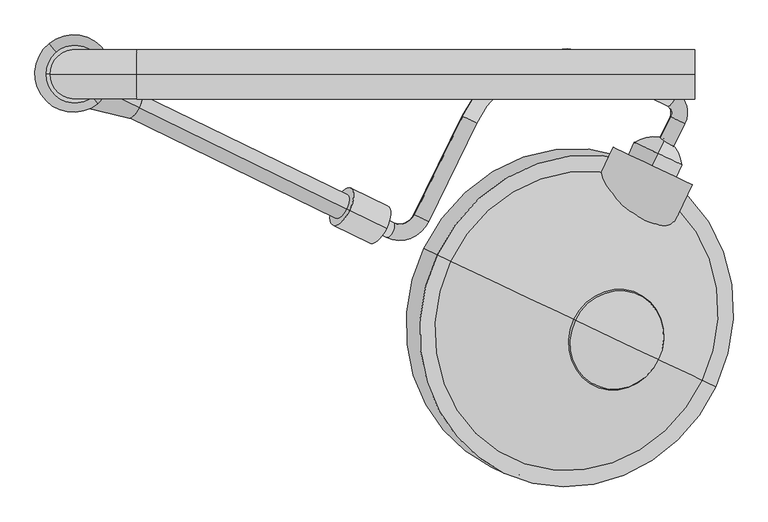
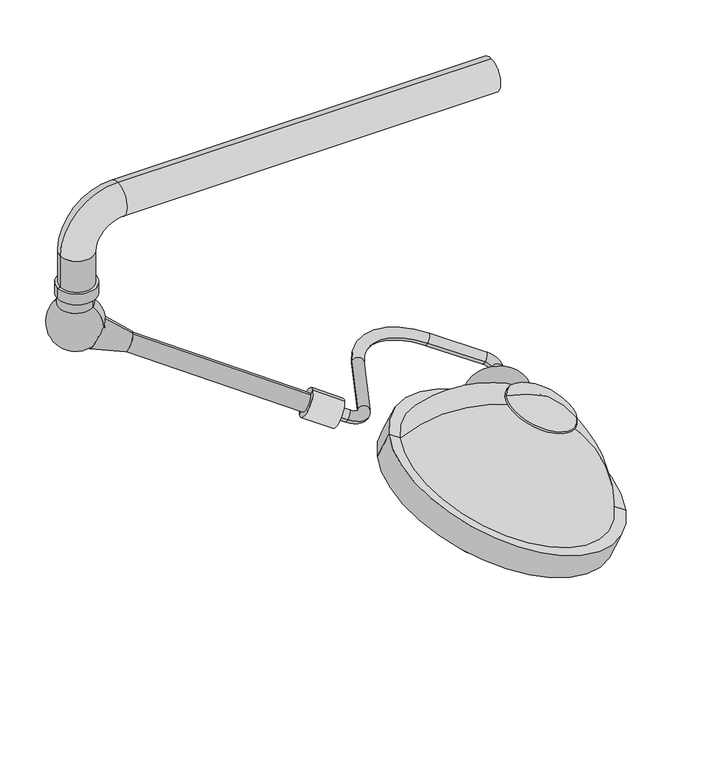
# IFC4 building model written with IfcOpenShell, lengths in millimetres: proxy geometry, M7490 - Light, Surg, Ceiling Mtd, Dual, Unequal Dia Heads : M7490 - Light, Surg, Ceiling Mtd, Dual, Unequal Dia Heads.
# Revit data of these elements (continued)
# Type "M7490 - Light, Surg, Ceiling Mtd, Dual, Unequal Dia Heads : M7490 - Light, Surg, Ceiling Mtd, Dual, Unequal Dia Heads"
#   JSN = "M7490"
#   Nomenclature = "Light, Surg, Ceiling Mtd, Dual, Unequal Dia Heads"
#   UTIL_1_WaterDrain = "-"
#   UTIL_2_Elec = "F"
#   UTIL_3_MedGas = "-"
#   UTIL_4_MiscGas = "-"
#   UTIL_5_NonMedGas = "-"
#   UTIL_6_Misc = "-"
#   Utility_6 = "-"
#   Utility_5 = "-"
#   Utility_4 = "-"
#   Utility_3 = "-"
#   Utility_2 = "F"
#   Utility_1 = "-"
#   Unit_Issue = "EA"
#   Price_Date = "0"
#   Nomenclature = "Light, Surg, Ceiling Mtd, Dual, Unequal Dia Heads"
#   NSN = "6530"
#   Location [instance default] = ""
#   JSN_Name = "M7490"
#   Hertz_swit = "0"
#   Hertz_dep = "-1"
#   Hertz = "60"
#   Desc = "Dual head surgical light ceiling mounted from a single pole. Unit has two lamp heads of differing sizes mounted on individual swing arms. Unit features multiple lighting pods in each lamp head, deep cavity illumination, color-corrected light, intensity control and sterilizable handles. Refer to the manufacturers' specifications for minimum ceiling heights and installation data. The database height dimension below refers to the height of the lamp head itself. The width and depth measurements are the larger of the two sums of the swing arm length and the head diameter. For use in general purpose surgical suites."
#   CAT_VA = "-"
#   CAT_Navy = "A"
#   CAT_IHS = "A"
#   CAT_Army = "A"
#   CAT_AF = "-"
#   BTUPerHour = "0"
#   Width_IN = 0
#   Weight_AV = 247
#   Watts2 = 0
#   Watts1 = 0
#   Volts2 = 0
#   Volts1 = 0
#   Phase2 = 0
#   Phase1 = 0
#   Height_IN = 0
#   Depth_IN = 0
#   Amps2 = 0
#   Amps1 = 0
#   finish [instance default] = none
# Element 1 (IfcBuildingElementProxy, "M7490 - Light, Surg, Ceiling Mtd, Dual, Unequal Dia Heads : M7490 - Light, Surg, Ceiling Mtd, Dual, Unequal Dia Heads")
#   Materials on its faces: "EquipSpace"
# Materials
#   "EquipSpace": class "Unassigned", colour RGB 221 217 195, transparency 0.5
